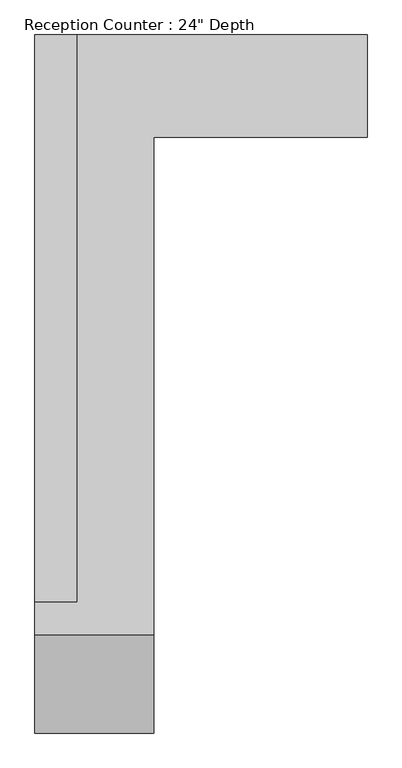
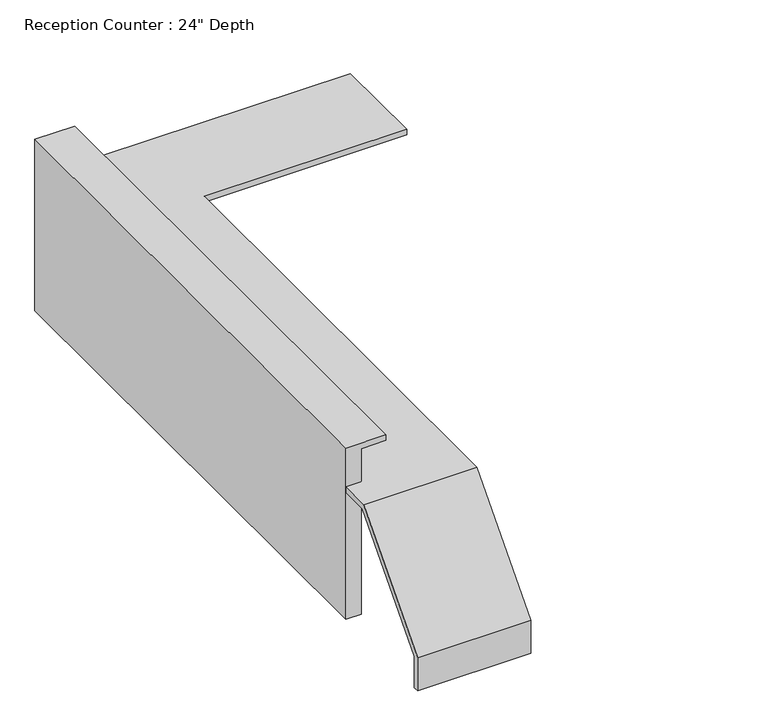
"""IFC4 building model written with IfcOpenShell, lengths in millimetres: furniture geometry."""

import ifcopenshell
import ifcopenshell.guid

model = None  # the IFC model being written
_history = None  # IfcOwnerHistory: only IFC2X3 demands one
_inside = {}  # id of a spatial element -> (the spatial element, [elements in it])
_under = {}  # id of a project, library or spatial element -> (it, [spatial elements below it])
_declared = {}  # id of a project -> (the project, [libraries it declares])
_typed = {}  # id of a type object -> (the type object, [elements of that type])
_made_of = {}  # id of a material, layer set ... -> (it, [elements and type objects made of it])


def new_model(schema):
    """Start an empty IFC model of exactly this schema.

    Asked for "IFC4X3", IfcOpenShell would pick the latest addendum, in which some entities
    have other attributes; the version numbers below select the first issue.
    IFC2X3 requires an IfcOwnerHistory on every rooted entity: one is made here for all.
    """
    global model, _history
    if schema == "IFC4X3":
        model = ifcopenshell.file(schema_version=(4, 3, 0, 0))
    else:
        model = ifcopenshell.file(schema=schema)
    _inside.clear()
    _under.clear()
    _declared.clear()
    _typed.clear()
    _made_of.clear()
    _history = None
    if model.schema == "IFC2X3":
        org = make("IfcOrganization", Name="unknown")
        user = make(
            "IfcPersonAndOrganization",
            ThePerson=make("IfcPerson", FamilyName="unknown"),
            TheOrganization=org,
        )
        app = make(
            "IfcApplication",
            ApplicationDeveloper=org,
            Version="unknown",
            ApplicationFullName="unknown",
            ApplicationIdentifier="unknown",
        )
        _history = make(
            "IfcOwnerHistory",
            OwningUser=user,
            OwningApplication=app,
            ChangeAction="ADDED",
            CreationDate=0,
        )
    return model


def make(cls, **values):
    """One entity of the class cls with the attributes given. An attribute that is None is left unset."""
    return model.create_entity(
        cls, **{name: value for name, value in values.items() if value is not None}
    )


def rooted(cls, **values):
    """An entity with a GlobalId (a new one), such as an element, a storey or a relation."""
    return make(cls, GlobalId=ifcopenshell.guid.new(), OwnerHistory=_history, **values)


def si_unit(unit_type, name, prefix=None):
    """IfcSIUnit, for example si_unit("LENGTHUNIT", "METRE", prefix="MILLI")."""
    return make("IfcSIUnit", UnitType=unit_type, Prefix=prefix, Name=name)


def assignment(units):
    """IfcUnitAssignment: the units of a project."""
    return None if units is None else make("IfcUnitAssignment", Units=units)


def point(xyz):
    """IfcCartesianPoint."""
    return None if xyz is None else make("IfcCartesianPoint", Coordinates=xyz)


def direction(xyz):
    """IfcDirection."""
    return None if xyz is None else make("IfcDirection", DirectionRatios=xyz)


def frame(location, z_axis=None, x_axis=None):
    """IfcAxis2Placement3D, a coordinate frame: its origin and axes. An axis left out is left unset."""
    return make(
        "IfcAxis2Placement3D",
        Location=point(location),
        Axis=direction(z_axis),
        RefDirection=direction(x_axis),
    )


def origin():
    """The frame at (0, 0, 0) with its axes left unset."""
    return frame((0.0, 0.0, 0.0))


def place(relative_to, where):
    """IfcLocalPlacement: puts the frame where relative to a parent placement (None: the world)."""
    return make(
        "IfcLocalPlacement", PlacementRelTo=relative_to, RelativePlacement=where
    )


def context(
    kind, dimensions, precision=None, world=None, true_north=None, identifier=None
):
    """IfcGeometricRepresentationContext, for example the 3D "Model" context."""
    return make(
        "IfcGeometricRepresentationContext",
        ContextIdentifier=identifier,
        ContextType=kind,
        CoordinateSpaceDimension=dimensions,
        Precision=precision,
        WorldCoordinateSystem=world,
        TrueNorth=true_north,
    )


def project(units=None, contexts=None):
    """IfcProject with its units and contexts."""
    return rooted(
        "IfcProject",
        Name="project",
        RepresentationContexts=contexts,
        UnitsInContext=assignment(units),
    )


def spatial(cls, under=None, at=None, **own):
    """A site, building, storey or space (cls), placed at a placement, below another one or the project."""
    s = rooted(cls, ObjectPlacement=at, **own)
    if under is not None:
        _under.setdefault(under.id(), (under, []))[1].append(s)
    return s


def polyline(points):
    """IfcPolyline through the points."""
    return make("IfcPolyline", Points=[point(p) for p in points])


def outline(outer, holes=None, kind="AREA"):
    """IfcArbitraryClosedProfileDef: a profile drawn as a closed curve; with holes, ...WithVoids."""
    if holes is None:
        return make("IfcArbitraryClosedProfileDef", ProfileType=kind, OuterCurve=outer)
    return make(
        "IfcArbitraryProfileDefWithVoids",
        ProfileType=kind,
        OuterCurve=outer,
        InnerCurves=holes,
    )


def extrude(swept, where, along, depth):
    """IfcExtrudedAreaSolid: the profile swept, set in the frame where, extruded along a direction by depth."""
    return make(
        "IfcExtrudedAreaSolid",
        SweptArea=swept,
        Position=where,
        ExtrudedDirection=direction(along),
        Depth=depth,
    )


def faces_of(points, faces, orient=None, outer=None):
    """IfcFace entities. A face is a list of loops; a loop is a list of indices into points, from 0.

    orient and outer hold one flag for each loop. By default every Orientation is true, the
    first loop of a face is its IfcFaceOuterBound and the others are IfcFaceBound.
    """
    made = []
    for i, loops in enumerate(faces):
        bounds = []
        for j, loop in enumerate(loops):
            is_outer = j == 0 if outer is None else outer[i][j]
            bounds.append(
                make(
                    "IfcFaceOuterBound" if is_outer else "IfcFaceBound",
                    Bound=make("IfcPolyLoop", Polygon=[points[k] for k in loop]),
                    Orientation=True if orient is None else orient[i][j],
                )
            )
        made.append(make("IfcFace", Bounds=bounds))
    return made


def faceted_brep(points, faces, orient=None, outer=None, voids=None):
    """IfcFacetedBrep: a solid bounded by flat faces; with voids (closed shells), ...WithVoids."""
    shared = [point(p) for p in points]
    hull = make("IfcClosedShell", CfsFaces=faces_of(shared, faces, orient, outer))
    if voids is None:
        return make("IfcFacetedBrep", Outer=hull)
    return make(
        "IfcFacetedBrepWithVoids",
        Outer=hull,
        Voids=[
            make(cls, CfsFaces=faces_of(shared, fs, o, b)) for cls, fs, o, b in voids
        ],
    )


def shape(context_of_items, identifier, shape_type, items):
    """IfcShapeRepresentation: the items that make up one representation, for example the "Body"."""
    return make(
        "IfcShapeRepresentation",
        ContextOfItems=context_of_items,
        RepresentationIdentifier=identifier,
        RepresentationType=shape_type,
        Items=items,
    )


def source(mapping_origin, context_of_items, identifier, shape_type, items):
    """IfcRepresentationMap: a shape defined once, which mapped items show again and again."""
    return make(
        "IfcRepresentationMap",
        MappingOrigin=mapping_origin,
        MappedRepresentation=shape(context_of_items, identifier, shape_type, items),
    )


def transform(
    local_origin,
    x_axis=None,
    y_axis=None,
    z_axis=None,
    scale=None,
    scale2=None,
    scale3=None,
    uniform=True,
):
    """IfcCartesianTransformationOperator3D, or its non-uniform kind. x_axis, y_axis, z_axis: its Axis1, 2, 3."""
    if uniform:
        return make(
            "IfcCartesianTransformationOperator3D",
            Axis1=direction(x_axis),
            Axis2=direction(y_axis),
            LocalOrigin=point(local_origin),
            Scale=scale,
            Axis3=direction(z_axis),
        )
    return make(
        "IfcCartesianTransformationOperator3DnonUniform",
        Axis1=direction(x_axis),
        Axis2=direction(y_axis),
        LocalOrigin=point(local_origin),
        Scale=scale,
        Axis3=direction(z_axis),
        Scale2=scale2,
        Scale3=scale3,
    )


def mapped(mapping_source, mapping_target):
    """IfcMappedItem: shows the shape of a source again, moved by a transform."""
    return make(
        "IfcMappedItem", MappingSource=mapping_source, MappingTarget=mapping_target
    )


def made_of(thing, what):
    """Note that an element or type object is made of a material, layer set ...; save() writes the relation."""
    if what is not None:
        _made_of.setdefault(what.id(), (what, []))[1].append(thing)
    return thing


def element(
    cls,
    number,
    at=None,
    inside=None,
    cuts=None,
    type_object=None,
    material=None,
    context=None,
    identifier="Body",
    shape_type=None,
    held_by="IfcProductDefinitionShape",
    body=None,
    shapes=None,
    **own,
):
    """One element of the class cls, such as IfcWall. Its Tag is "e" and its number.

    at: its placement. inside: the storey or other place that contains it. cuts: it is an
    opening in that element (IfcRelVoidsElement). A single representation is given by context,
    identifier, shape_type and body (its items); several are given by shapes. held_by: the class
    of the entity that holds the representations. save() writes the other relations.
    """
    e = rooted(cls, Tag="e%d" % number, ObjectPlacement=at, **own)
    if body is not None:
        shapes = [shape(context, identifier, shape_type, body)]
    if shapes is not None:
        e.Representation = make(held_by, Representations=shapes)
    if inside is not None:
        _inside.setdefault(inside.id(), (inside, []))[1].append(e)
    if cuts is not None:
        rooted(
            "IfcRelVoidsElement", RelatingBuildingElement=cuts, RelatedOpeningElement=e
        )
    if type_object is not None:
        _typed.setdefault(type_object.id(), (type_object, []))[1].append(e)
    return made_of(e, material)


def aggregate(whole, parts):
    """IfcRelAggregates: a whole, such as a stair, and the parts it consists of."""
    return rooted("IfcRelAggregates", RelatingObject=whole, RelatedObjects=parts)


def save(model, path):
    """Write the relations noted so far, then the file.

    IfcRelAggregates (storeys below a building ...), IfcRelContainedInSpatialStructure (elements
    in a storey), IfcRelDefinesByType, IfcRelAssociatesMaterial and IfcRelDeclares: one each for
    every whole, place, type object, material and project.
    """
    for whole, parts in _under.values():
        aggregate(whole, parts)
    for where, things in _inside.values():
        rooted(
            "IfcRelContainedInSpatialStructure",
            RelatedElements=things,
            RelatingStructure=where,
        )
    for kind, things in _typed.values():
        rooted("IfcRelDefinesByType", RelatedObjects=things, RelatingType=kind)
    for what, things in _made_of.values():
        rooted("IfcRelAssociatesMaterial", RelatedObjects=things, RelatingMaterial=what)
    for by, libraries in _declared.values():
        rooted("IfcRelDeclares", RelatingContext=by, RelatedDefinitions=libraries)
    model.write(path)


def furniture_35f6b429(model_context):
    return source(origin(), model_context, "Body", "SolidModel", [
        extrude(outline(polyline([(0.0, -1302.0622951), (0.0, -1200.4622951), (1143.0, -1200.4622951), (1143.0, -1041.7122951), (1181.1, -1041.7122951), (1181.1, -1302.0622951), (0.0, -1302.0622951)])), frame((0.0, -3511.55, 0.0), z_axis=(0.0, 1.0, 0.0), x_axis=(0.0, 0.0, 1.0)), (0.0, 0.0, 1.0), 3511.55),
        faceted_brep([(755.3377049, 0.0, 914.4), (-1200.4622951, 0.0, 914.4), (-1200.4622951, -3511.55, 914.4), (-1302.0622951, -3511.55, 914.4), (-1302.0622951, -3714.75, 914.4), (-565.4622951, -3714.75, 914.4), (-565.4622951, -635.0, 914.4), (755.3377049, -635.0, 914.4), (755.3377049, 0.0, 876.3), (755.3377049, -635.0, 876.3), (-565.4622951, -635.0, 876.3), (-565.4622951, -3697.6405829, 876.3), (-1302.0622951, -3697.6405829, 876.3), (-1302.0622951, -3511.55, 876.3), (-1200.4622951, -3511.55, 876.3), (-1200.4622951, 0.0, 876.3), (-565.4622951, -4324.35, 228.6), (-565.4622951, -4324.35, 0.0), (-565.4622951, -4286.25, 0.0), (-565.4622951, -4286.25, 214.1144058), (-1302.0622951, -4324.35, 228.6), (-1302.0622951, -4286.25, 214.1144058), (-1302.0622951, -4286.25, 0.0), (-1302.0622951, -4324.35, 0.0)], [[[0, 1, 2, 3, 4, 5, 6, 7]], [[8, 9, 10, 11, 12, 13, 14, 15]], [[1, 0, 8, 15]], [[2, 1, 15, 14]], [[6, 5, 16, 17, 18, 19, 11, 10]], [[7, 6, 10, 9]], [[0, 7, 9, 8]], [[20, 4, 3, 13, 12, 21, 22, 23]], [[4, 20, 16, 5]], [[21, 12, 11, 19]], [[22, 21, 19, 18]], [[23, 22, 18, 17]], [[20, 23, 17, 16]], [[13, 3, 2, 14]]]),
    ])


if __name__ == "__main__":
    model = new_model("IFC4")
    model_context = context("Model", 3, world=origin())
    ifc_project = project(units=[si_unit("LENGTHUNIT", "METRE", prefix="MILLI")], contexts=[model_context])
    site = spatial("IfcSite", under=ifc_project)
    building = spatial("IfcBuilding", under=site)
    placement = place(None, origin())
    furniture_shape = furniture_35f6b429(model_context)
    element("IfcFurniture", 1, ObjectType="Reception Counter : 24\" Depth", at=placement, inside=building, context=model_context, shape_type="MappedRepresentation", body=[
        mapped(furniture_shape, transform((0.0, 0.0, 0.0), x_axis=(1.0, 0.0, 0.0), y_axis=(0.0, 1.0, 0.0), z_axis=(0.0, 0.0, 1.0))),
    ])
    save(model, "model.ifc")

# Revit data of these elements
# Type "Reception Counter : 24\" Depth"
#   Assembly Code = "C1030400"
#   X [instance default] = 2' - 0"
#   Wall Thickness [instance default] = 0' - 4"
#   Transaction Counter Depth [instance default] = 0' - 6 1/4"
#   Transaction Counter Rise [instance default] = 0' - 9"
#   Counter Thickness = 0' - 1 1/2"
#   Depth = 2' - 1"
#   Height = 3' - 0"
#   Length - Leg 1 [instance default] = 6' - 5"
#   Length - Leg 2 [instance default] = 12' - 3"
#   Transaction Counter Material = Concrete Board Form
#   Counter Top Material = Laminate, Ivory, Matte
#   Default Elevation = 0
# Element 1 (IfcFurniture, "Reception Counter : 24\" Depth")
#   Length - Leg 2 = 12' - 2 1/4"
#   Materials on its faces: "Laminate, Ivory, Matte", "Concrete Board Form"
# Materials
#   "Concrete Board Form": class "Concrete", colour RGB 131 127 122, transparency 0, Description = "Lightweight concrete", Cost = 0
#   "Laminate, Ivory, Matte": class "Plastic", colour RGB 247 247 239, transparency 0, Description = "Plastic Laminate - Ivory, Matte", Cost = 0
